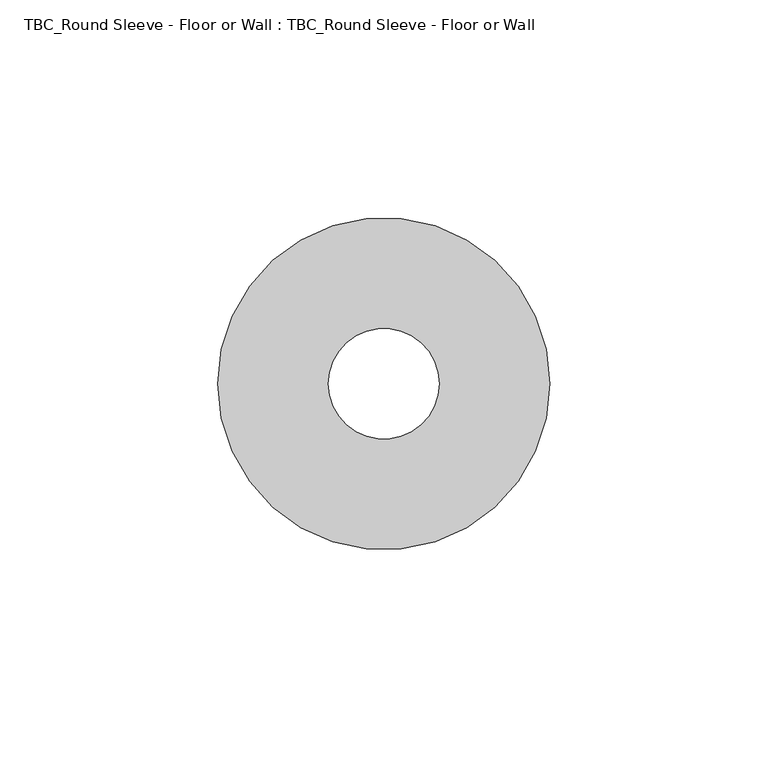
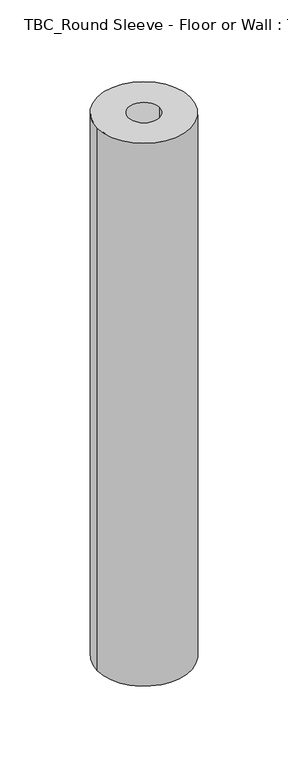
"""IFC4 building model written with IfcOpenShell, lengths in millimetres: proxy geometry, TBC_Round Sleeve - Floor or Wall : TBC_Round Sleeve - Floor or Wall."""

from ifc_helpers import new_model, si_unit, point, frame, origin, origin_2d, place, context, project, spatial, circle_curve, trimmed, segment, composite_curve, outline, extrude, source, transform, mapped, element, save


def tbc_round_sleeve_floor_or_wall_tbc_round_sleeve_floor_or_a8df504e(model_context):
    return source(origin(), model_context, "Body", "SweptSolid", [
        extrude(outline(composite_curve([segment(trimmed(circle_curve(origin_2d(), 38.1), [point((-38.1, 0.0))], [point((38.1, 0.0))], False, "CARTESIAN"), True, "CONTINUOUS"), segment(trimmed(circle_curve(origin_2d(), 38.1), [point((38.1, 0.0))], [point((-38.1, 0.0))], False, "CARTESIAN"), True, "CONTINUOUS")], self_intersect=False), holes=[composite_curve([segment(trimmed(circle_curve(origin_2d(), 12.7), [point((-12.7, 0.0))], [point((12.7, 0.0))], True, "CARTESIAN"), True, "CONTINUOUS"), segment(trimmed(circle_curve(origin_2d(), 12.7), [point((12.7, 0.0))], [point((-12.7, 0.0))], True, "CARTESIAN"), True, "CONTINUOUS")], self_intersect=False)]), frame((0.0, 0.0, -469.9), z_axis=(0.0, 0.0, 1.0), x_axis=(1.0, 0.0, 0.0)), (0.0, 0.0, 1.0), 469.9),
    ])


if __name__ == "__main__":
    model = new_model("IFC4")
    model_context = context("Model", 3, world=origin())
    ifc_project = project(units=[si_unit("LENGTHUNIT", "METRE", prefix="MILLI")], contexts=[model_context])
    site = spatial("IfcSite", under=ifc_project)
    building = spatial("IfcBuilding", under=site)
    placement = place(None, origin())
    tbc_round_sleeve_floor_or_wall_tbc_round_sleeve_floor_or_shape = tbc_round_sleeve_floor_or_wall_tbc_round_sleeve_floor_or_a8df504e(model_context)
    element("IfcBuildingElementProxy", 1, Name="TBC_Round Sleeve - Floor or Wall : TBC_Round Sleeve - Floor or Wall", ObjectType="TBC_Round Sleeve - Floor or Wall : TBC_Round Sleeve - Floor or Wall", at=placement, inside=building, context=model_context, shape_type="MappedRepresentation", body=[
        mapped(tbc_round_sleeve_floor_or_wall_tbc_round_sleeve_floor_or_shape, transform((0.0, 0.0, 0.0), x_axis=(1.0, 0.0, 0.0), y_axis=(0.0, 1.0, 0.0), z_axis=(0.0, 0.0, 1.0))),
    ])
    save(model, "model.ifc")

# Revit data of these elements
# Type "TBC_Round Sleeve - Floor or Wall : TBC_Round Sleeve - Floor or Wall"
#   Tag Dimension [instance default] = ""
#   MEP Type [instance default] = ""
#   MEP Element [instance default] = ""
#   MEP Category [instance default] = ""
#   Host Element Type [instance default] = ""
#   Host Element Id [instance default] = ""
#   Host Element Category [instance default] = ""
#   Control Line Y [instance default] = ""
#   Control Line X [instance default] = ""
#   Sleeve Radius [instance default] = 1' - 0"
#   Sleeve Edge [instance default] = 1' - 2"
#   Sleeve Depth [instance default] = 3' - 0"
#   Distance Y [instance default] = 0' - 0"
#   Distance X [instance default] = 0' - 0"
#   Default Elevation = 0
# Element 1 (IfcBuildingElementProxy, "TBC_Round Sleeve - Floor or Wall : TBC_Round Sleeve - Floor or Wall")
#   Sleeve Radius = 0' - 1"
#   Sleeve Edge = 0' - 3"
#   Sleeve Depth = 1' - 6 1/2"
